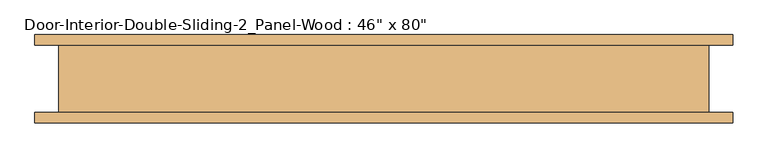
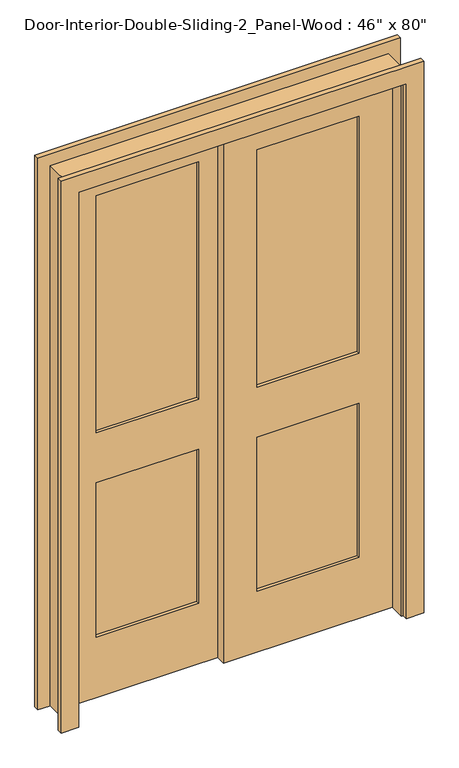
"""IFC4 building model written with IfcOpenShell, lengths in millimetres: door geometry."""

from ifc_helpers import new_model, si_unit, frame, origin, place, context, project, spatial, polyline, outline, extrude, source, transform, mapped, element, save


def door_0fd0fe05(model_context):
    return source(origin(), model_context, "Body", "SweptSolid", [
        extrude(outline(polyline([(463.55, 2.1166667), (95.25, 2.1166667), (95.25, 13.7583333), (463.55, 13.7583333), (463.55, 2.1166667)])), frame((0.0, 0.0, 1009.65), z_axis=(0.0, 0.0, 1.0), x_axis=(1.0, 0.0, 0.0)), (0.0, 0.0, 1.0), 903.2875),
        extrude(outline(polyline([(463.55, 2.1166667), (95.25, 2.1166667), (95.25, 13.7583333), (463.55, 13.7583333), (463.55, 2.1166667)])), frame((0.0, 0.0, 231.775), z_axis=(0.0, 0.0, 1.0), x_axis=(1.0, 0.0, 0.0)), (0.0, 0.0, 1.0), 587.375),
        extrude(outline(polyline([(2032.0, -25.4), (0.0, -25.4), (0.0, 584.2), (2032.0, 584.2), (2032.0, -25.4)]), holes=[polyline([(1912.9375, 95.25), (1912.9375, 463.55), (1009.65, 463.55), (1009.65, 95.25), (1912.9375, 95.25)]), polyline([(819.15, 95.25), (819.15, 463.55), (231.775, 463.55), (231.775, 95.25), (819.15, 95.25)])]), frame((0.0, -9.525, 0.0), z_axis=(0.0, 1.0, 0.0), x_axis=(0.0, 0.0, 1.0)), (0.0, 0.0, 1.0), 34.925),
        extrude(outline(polyline([(-95.25, 37.0416667), (-463.55, 37.0416667), (-463.55, 48.6833333), (-95.25, 48.6833333), (-95.25, 37.0416667)])), frame((0.0, 0.0, 1009.65), z_axis=(0.0, 0.0, 1.0), x_axis=(1.0, 0.0, 0.0)), (0.0, 0.0, 1.0), 903.2875),
        extrude(outline(polyline([(-95.25, 37.0416667), (-463.55, 37.0416667), (-463.55, 48.6833333), (-95.25, 48.6833333), (-95.25, 37.0416667)])), frame((0.0, 0.0, 231.775), z_axis=(0.0, 0.0, 1.0), x_axis=(1.0, 0.0, 0.0)), (0.0, 0.0, 1.0), 587.375),
        extrude(outline(polyline([(2032.0, -584.2), (0.0, -584.2), (0.0, 25.4), (2032.0, 25.4), (2032.0, -584.2)]), holes=[polyline([(1912.9375, -463.55), (1912.9375, -95.25), (1009.65, -95.25), (1009.65, -463.55), (1912.9375, -463.55)]), polyline([(819.15, -463.55), (819.15, -95.25), (231.775, -95.25), (231.775, -463.55), (819.15, -463.55)])]), frame((0.0, 25.4, 0.0), z_axis=(0.0, 1.0, 0.0), x_axis=(0.0, 0.0, 1.0)), (0.0, 0.0, 1.0), 34.925),
        extrude(outline(polyline([(0.0, 584.2), (0.0, 609.6), (2057.4, 609.6), (2057.4, -609.6), (0.0, -609.6), (0.0, -584.2), (2032.0, -584.2), (2032.0, 584.2), (0.0, 584.2)])), frame((0.0, -66.675, 0.0), z_axis=(0.0, 1.0, 0.0), x_axis=(0.0, 0.0, 1.0)), (0.0, 0.0, 1.0), 127.0),
        extrude(outline(polyline([(0.0, 590.55), (0.0, 654.05), (2101.85, 654.05), (2101.85, -654.05), (0.0, -654.05), (0.0, -590.55), (2038.35, -590.55), (2038.35, 590.55), (0.0, 590.55)])), frame((0.0, -85.725, 0.0), z_axis=(0.0, 1.0, 0.0), x_axis=(0.0, 0.0, 1.0)), (0.0, 0.0, 1.0), 19.05),
        extrude(outline(polyline([(0.0, 590.55), (0.0, 654.05), (2101.85, 654.05), (2101.85, -654.05), (0.0, -654.05), (0.0, -590.55), (2038.35, -590.55), (2038.35, 590.55), (0.0, 590.55)])), frame((0.0, 60.325, 0.0), z_axis=(0.0, 1.0, 0.0), x_axis=(0.0, 0.0, 1.0)), (0.0, 0.0, 1.0), 19.05),
    ])


if __name__ == "__main__":
    model = new_model("IFC4")
    model_context = context("Model", 3, world=origin())
    ifc_project = project(units=[si_unit("LENGTHUNIT", "METRE", prefix="MILLI")], contexts=[model_context])
    site = spatial("IfcSite", under=ifc_project)
    building = spatial("IfcBuilding", under=site)
    placement = place(None, origin())
    door_shape = door_0fd0fe05(model_context)
    element("IfcDoor", 1, ObjectType="Door-Interior-Double-Sliding-2_Panel-Wood : 46\" x 80\"", at=placement, inside=building, context=model_context, shape_type="MappedRepresentation", body=[
        mapped(door_shape, transform((0.0, 0.0, 0.0), x_axis=(1.0, 0.0, 0.0), y_axis=(0.0, 1.0, 0.0), z_axis=(0.0, 0.0, 1.0))),
    ])
    save(model, "model.ifc")

# Revit data of these elements
# Type "Door-Interior-Double-Sliding-2_Panel-Wood : 46\" x 80\""
#   Type Mark = "26"
#   Assembly Code = "C1020300"
#   Analytic Construction = "Wooden"
#   Top Rail = 0' - 4 11/16"
#   Thickness = 0' - 1 3/8"
#   Thermal Resistance (R) = 2.5876 (h·ft²·°F)/BTU
#   Stiles = 0' - 4 3/4"
#   Rough Width = 4' - 0"
#   Rough Height = 6' - 9"
#   Lock Rail = 0' - 7 1/2"
#   Height = 6' - 8"
#   Width = 3' - 10"
#   Heat Transfer Coefficient (U) = 0.3865 BTU/(h·ft²·°F)
#   Bottom Rail = 0' - 9 1/8"
#   Trim Material = Cherry
#   Panel Material = Cherry
#   Frame Material = Cherry
#   Visual Light Transmittance = 0
#   Solar Heat Gain Coefficient = 0
#   Wall Closure = (empty or 0)
#   Function = (empty or 0)
# Element 1 (IfcDoor, "Door-Interior-Double-Sliding-2_Panel-Wood : 46\" x 80\"")
#   Materials on its faces: "Cherry"
# Materials
#   "Cherry": class "Wood", colour RGB 226 177 128, transparency 0, Description = "Prunus Serotina", Cost = 0
